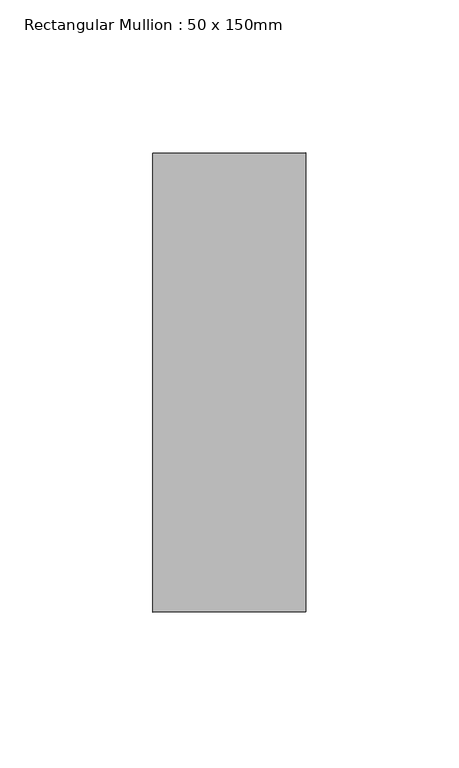
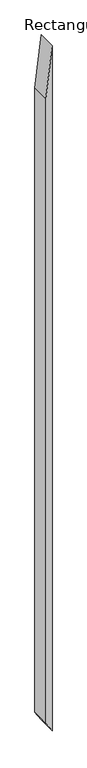
"""IFC4 building model written with IfcOpenShell, lengths in millimetres: member geometry, Rectangular Mullion : 50 x 150mm."""

import ifcopenshell
import ifcopenshell.guid

model = None  # the IFC model being written
_history = None  # IfcOwnerHistory: only IFC2X3 demands one
_inside = {}  # id of a spatial element -> (the spatial element, [elements in it])
_under = {}  # id of a project, library or spatial element -> (it, [spatial elements below it])
_declared = {}  # id of a project -> (the project, [libraries it declares])
_typed = {}  # id of a type object -> (the type object, [elements of that type])
_made_of = {}  # id of a material, layer set ... -> (it, [elements and type objects made of it])


def new_model(schema):
    """Start an empty IFC model of exactly this schema.

    Asked for "IFC4X3", IfcOpenShell would pick the latest addendum, in which some entities
    have other attributes; the version numbers below select the first issue.
    IFC2X3 requires an IfcOwnerHistory on every rooted entity: one is made here for all.
    """
    global model, _history
    if schema == "IFC4X3":
        model = ifcopenshell.file(schema_version=(4, 3, 0, 0))
    else:
        model = ifcopenshell.file(schema=schema)
    _inside.clear()
    _under.clear()
    _declared.clear()
    _typed.clear()
    _made_of.clear()
    _history = None
    if model.schema == "IFC2X3":
        org = make("IfcOrganization", Name="unknown")
        user = make(
            "IfcPersonAndOrganization",
            ThePerson=make("IfcPerson", FamilyName="unknown"),
            TheOrganization=org,
        )
        app = make(
            "IfcApplication",
            ApplicationDeveloper=org,
            Version="unknown",
            ApplicationFullName="unknown",
            ApplicationIdentifier="unknown",
        )
        _history = make(
            "IfcOwnerHistory",
            OwningUser=user,
            OwningApplication=app,
            ChangeAction="ADDED",
            CreationDate=0,
        )
    return model


def make(cls, **values):
    """One entity of the class cls with the attributes given. An attribute that is None is left unset."""
    return model.create_entity(
        cls, **{name: value for name, value in values.items() if value is not None}
    )


def rooted(cls, **values):
    """An entity with a GlobalId (a new one), such as an element, a storey or a relation."""
    return make(cls, GlobalId=ifcopenshell.guid.new(), OwnerHistory=_history, **values)


def si_unit(unit_type, name, prefix=None):
    """IfcSIUnit, for example si_unit("LENGTHUNIT", "METRE", prefix="MILLI")."""
    return make("IfcSIUnit", UnitType=unit_type, Prefix=prefix, Name=name)


def assignment(units):
    """IfcUnitAssignment: the units of a project."""
    return None if units is None else make("IfcUnitAssignment", Units=units)


def point(xyz):
    """IfcCartesianPoint."""
    return None if xyz is None else make("IfcCartesianPoint", Coordinates=xyz)


def direction(xyz):
    """IfcDirection."""
    return None if xyz is None else make("IfcDirection", DirectionRatios=xyz)


def frame(location, z_axis=None, x_axis=None):
    """IfcAxis2Placement3D, a coordinate frame: its origin and axes. An axis left out is left unset."""
    return make(
        "IfcAxis2Placement3D",
        Location=point(location),
        Axis=direction(z_axis),
        RefDirection=direction(x_axis),
    )


def origin():
    """The frame at (0, 0, 0) with its axes left unset."""
    return frame((0.0, 0.0, 0.0))


def place(relative_to, where):
    """IfcLocalPlacement: puts the frame where relative to a parent placement (None: the world)."""
    return make(
        "IfcLocalPlacement", PlacementRelTo=relative_to, RelativePlacement=where
    )


def context(
    kind, dimensions, precision=None, world=None, true_north=None, identifier=None
):
    """IfcGeometricRepresentationContext, for example the 3D "Model" context."""
    return make(
        "IfcGeometricRepresentationContext",
        ContextIdentifier=identifier,
        ContextType=kind,
        CoordinateSpaceDimension=dimensions,
        Precision=precision,
        WorldCoordinateSystem=world,
        TrueNorth=true_north,
    )


def project(units=None, contexts=None):
    """IfcProject with its units and contexts."""
    return rooted(
        "IfcProject",
        Name="project",
        RepresentationContexts=contexts,
        UnitsInContext=assignment(units),
    )


def spatial(cls, under=None, at=None, **own):
    """A site, building, storey or space (cls), placed at a placement, below another one or the project."""
    s = rooted(cls, ObjectPlacement=at, **own)
    if under is not None:
        _under.setdefault(under.id(), (under, []))[1].append(s)
    return s


def polyline(points):
    """IfcPolyline through the points."""
    return make("IfcPolyline", Points=[point(p) for p in points])


def outline(outer, holes=None, kind="AREA"):
    """IfcArbitraryClosedProfileDef: a profile drawn as a closed curve; with holes, ...WithVoids."""
    if holes is None:
        return make("IfcArbitraryClosedProfileDef", ProfileType=kind, OuterCurve=outer)
    return make(
        "IfcArbitraryProfileDefWithVoids",
        ProfileType=kind,
        OuterCurve=outer,
        InnerCurves=holes,
    )


def extrude(swept, where, along, depth):
    """IfcExtrudedAreaSolid: the profile swept, set in the frame where, extruded along a direction by depth."""
    return make(
        "IfcExtrudedAreaSolid",
        SweptArea=swept,
        Position=where,
        ExtrudedDirection=direction(along),
        Depth=depth,
    )


def shape(context_of_items, identifier, shape_type, items):
    """IfcShapeRepresentation: the items that make up one representation, for example the "Body"."""
    return make(
        "IfcShapeRepresentation",
        ContextOfItems=context_of_items,
        RepresentationIdentifier=identifier,
        RepresentationType=shape_type,
        Items=items,
    )


def source(mapping_origin, context_of_items, identifier, shape_type, items):
    """IfcRepresentationMap: a shape defined once, which mapped items show again and again."""
    return make(
        "IfcRepresentationMap",
        MappingOrigin=mapping_origin,
        MappedRepresentation=shape(context_of_items, identifier, shape_type, items),
    )


def transform(
    local_origin,
    x_axis=None,
    y_axis=None,
    z_axis=None,
    scale=None,
    scale2=None,
    scale3=None,
    uniform=True,
):
    """IfcCartesianTransformationOperator3D, or its non-uniform kind. x_axis, y_axis, z_axis: its Axis1, 2, 3."""
    if uniform:
        return make(
            "IfcCartesianTransformationOperator3D",
            Axis1=direction(x_axis),
            Axis2=direction(y_axis),
            LocalOrigin=point(local_origin),
            Scale=scale,
            Axis3=direction(z_axis),
        )
    return make(
        "IfcCartesianTransformationOperator3DnonUniform",
        Axis1=direction(x_axis),
        Axis2=direction(y_axis),
        LocalOrigin=point(local_origin),
        Scale=scale,
        Axis3=direction(z_axis),
        Scale2=scale2,
        Scale3=scale3,
    )


def mapped(mapping_source, mapping_target):
    """IfcMappedItem: shows the shape of a source again, moved by a transform."""
    return make(
        "IfcMappedItem", MappingSource=mapping_source, MappingTarget=mapping_target
    )


def made_of(thing, what):
    """Note that an element or type object is made of a material, layer set ...; save() writes the relation."""
    if what is not None:
        _made_of.setdefault(what.id(), (what, []))[1].append(thing)
    return thing


def element(
    cls,
    number,
    at=None,
    inside=None,
    cuts=None,
    type_object=None,
    material=None,
    context=None,
    identifier="Body",
    shape_type=None,
    held_by="IfcProductDefinitionShape",
    body=None,
    shapes=None,
    **own,
):
    """One element of the class cls, such as IfcWall. Its Tag is "e" and its number.

    at: its placement. inside: the storey or other place that contains it. cuts: it is an
    opening in that element (IfcRelVoidsElement). A single representation is given by context,
    identifier, shape_type and body (its items); several are given by shapes. held_by: the class
    of the entity that holds the representations. save() writes the other relations.
    """
    e = rooted(cls, Tag="e%d" % number, ObjectPlacement=at, **own)
    if body is not None:
        shapes = [shape(context, identifier, shape_type, body)]
    if shapes is not None:
        e.Representation = make(held_by, Representations=shapes)
    if inside is not None:
        _inside.setdefault(inside.id(), (inside, []))[1].append(e)
    if cuts is not None:
        rooted(
            "IfcRelVoidsElement", RelatingBuildingElement=cuts, RelatedOpeningElement=e
        )
    if type_object is not None:
        _typed.setdefault(type_object.id(), (type_object, []))[1].append(e)
    return made_of(e, material)


def aggregate(whole, parts):
    """IfcRelAggregates: a whole, such as a stair, and the parts it consists of."""
    return rooted("IfcRelAggregates", RelatingObject=whole, RelatedObjects=parts)


def save(model, path):
    """Write the relations noted so far, then the file.

    IfcRelAggregates (storeys below a building ...), IfcRelContainedInSpatialStructure (elements
    in a storey), IfcRelDefinesByType, IfcRelAssociatesMaterial and IfcRelDeclares: one each for
    every whole, place, type object, material and project.
    """
    for whole, parts in _under.values():
        aggregate(whole, parts)
    for where, things in _inside.values():
        rooted(
            "IfcRelContainedInSpatialStructure",
            RelatedElements=things,
            RelatingStructure=where,
        )
    for kind, things in _typed.values():
        rooted("IfcRelDefinesByType", RelatedObjects=things, RelatingType=kind)
    for what, things in _made_of.values():
        rooted("IfcRelAssociatesMaterial", RelatedObjects=things, RelatingMaterial=what)
    for by, libraries in _declared.values():
        rooted("IfcRelDeclares", RelatingContext=by, RelatedDefinitions=libraries)
    model.write(path)


def rectangular_mullion_50_x_150mm_1c2bc1f0(model_context):
    return source(origin(), model_context, "Body", "SweptSolid", [
        extrude(outline(polyline([(0.0, 0.0), (-433.116945, -50.0), (-5688.9606912, -50.0), (-5767.4004184, 0.0), (0.0, 0.0)])), frame((0.0, -75.0, 0.0), z_axis=(0.0, 1.0, 0.0), x_axis=(0.0, 0.0, 1.0)), (0.0, 0.0, 1.0), 150.0),
    ])


if __name__ == "__main__":
    model = new_model("IFC4")
    model_context = context("Model", 3, world=origin())
    ifc_project = project(units=[si_unit("LENGTHUNIT", "METRE", prefix="MILLI")], contexts=[model_context])
    site = spatial("IfcSite", under=ifc_project)
    building = spatial("IfcBuilding", under=site)
    placement = place(None, origin())
    rectangular_mullion_50_x_150mm_shape = rectangular_mullion_50_x_150mm_1c2bc1f0(model_context)
    element("IfcMember", 1, ObjectType="Rectangular Mullion : 50 x 150mm", at=placement, inside=building, context=model_context, shape_type="MappedRepresentation", body=[
        mapped(rectangular_mullion_50_x_150mm_shape, transform((0.0, 0.0, 0.0), x_axis=(1.0, 0.0, 0.0), y_axis=(0.0, 1.0, 0.0), z_axis=(0.0, 0.0, 1.0))),
    ])
    save(model, "model.ifc")

# Revit data of these elements
# Type "Rectangular Mullion : 50 x 150mm"
#   built-in parameter 1007304 = 0.492126 (stored number, unit not read)
#   built-in parameter 1007301 = 0.082021 (stored number, unit not read)
#   built-in parameter 1007300 = 0.082021 (stored number, unit not read)
# Element 1 (IfcMember, "Rectangular Mullion : 50 x 150mm")
#   Materials on its faces: "Metal - Aluminium"
# Materials
#   "Metal - Aluminium": class "Metal", colour RGB 247 247 247, transparency 0
